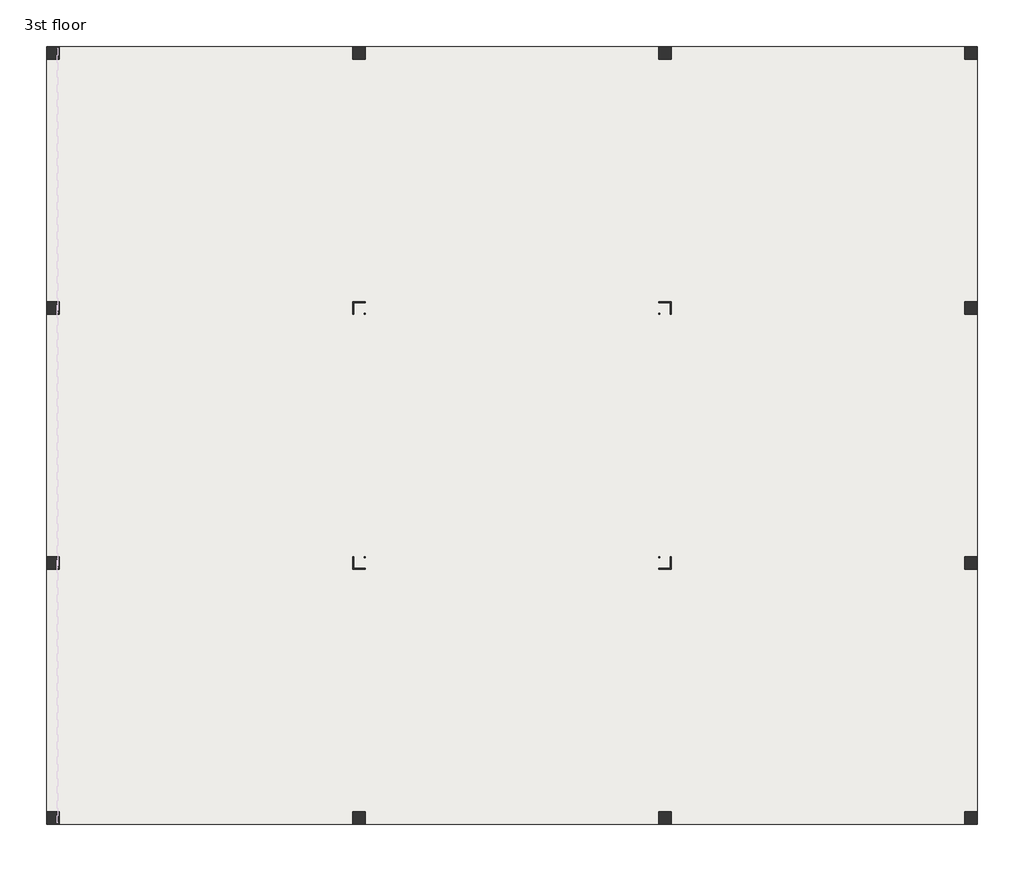
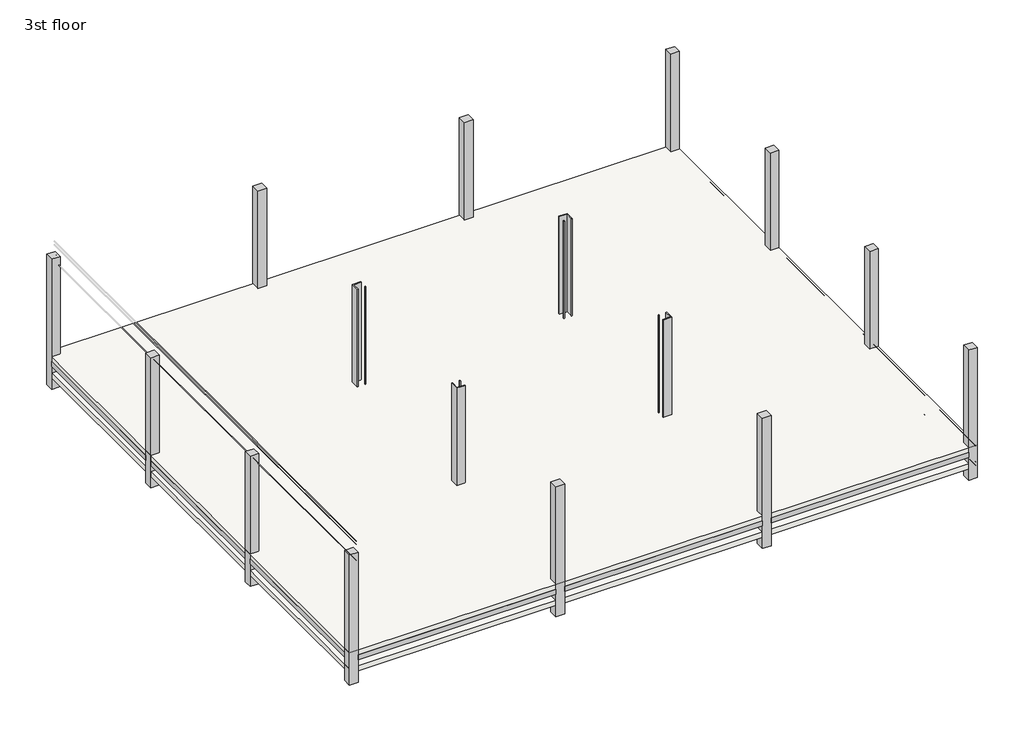
# One storey, part 1 of 2: 24 beams, 16 columns, 2 slabs.
"""IFC4 building model written with IfcOpenShell, lengths in millimetres."""

from ifc_helpers import new_model, si_unit, frame, origin, place, context, project, spatial, polyline, outline, extrude, faceted_brep, element, save

model = new_model("IFC4")

# Units and contexts
model_context = context("Model", 3, world=origin())
ifc_project = project(units=[si_unit("LENGTHUNIT", "METRE", prefix="MILLI")], contexts=[model_context])

# Site, building, storey
site = spatial("IfcSite", under=ifc_project)
building = spatial("IfcBuilding", under=site)
storey = spatial("IfcBuildingStorey", under=building, Name="3st floor", Elevation=12000.0)

# Beams
placement = place(None, origin())
element("IfcBeam", 1, ObjectType="Concrete-Rectangular Beam : 250 x 300mm", at=placement, inside=storey, context=model_context, shape_type="SweptSolid", body=[
    extrude(outline(polyline([(-8833.7181639, -5693.2383613), (-8833.7181639, -5443.2383613), (-3083.7181639, -5443.2383613), (-3083.7181639, -5693.2383613), (-8833.7181639, -5693.2383613)])), frame((0.0, 0.0, 11700.0), z_axis=(0.0, 0.0, 1.0), x_axis=(1.0, 0.0, 0.0)), (0.0, 0.0, 1.0), 150.0),
])
element("IfcBeam", 2, ObjectType="Concrete-Rectangular Beam : 250 x 300mm", at=placement, inside=storey, context=model_context, shape_type="SweptSolid", body=[
    extrude(outline(polyline([(-2833.7181639, -5693.2383613), (-2833.7181639, -5443.2383613), (2916.2818361, -5443.2383613), (2916.2818361, -5693.2383613), (-2833.7181639, -5693.2383613)])), frame((0.0, 0.0, 11700.0), z_axis=(0.0, 0.0, 1.0), x_axis=(1.0, 0.0, 0.0)), (0.0, 0.0, 1.0), 150.0),
])
element("IfcBeam", 3, ObjectType="Concrete-Rectangular Beam : 250 x 300mm", at=placement, inside=storey, context=model_context, shape_type="SweptSolid", body=[
    extrude(outline(polyline([(3166.2818361, -5693.2383613), (3166.2818361, -5443.2383613), (8916.2818361, -5443.2383613), (8916.2818361, -5693.2383613), (3166.2818361, -5693.2383613)])), frame((0.0, 0.0, 11700.0), z_axis=(0.0, 0.0, 1.0), x_axis=(1.0, 0.0, 0.0)), (0.0, 0.0, 1.0), 150.0),
])
element("IfcBeam", 4, ObjectType="Concrete-Rectangular Beam : 250 x 300mm", at=placement, inside=storey, context=model_context, shape_type="SweptSolid", body=[
    extrude(outline(polyline([(-8833.7181639, -10443.2383613), (-9083.7181639, -10443.2383613), (-9083.7181639, -5693.2383613), (-8833.7181639, -5693.2383613), (-8833.7181639, -10443.2383613)])), frame((0.0, 0.0, 11700.0), z_axis=(0.0, 0.0, 1.0), x_axis=(1.0, 0.0, 0.0)), (0.0, 0.0, 1.0), 150.0),
])
element("IfcBeam", 5, ObjectType="Concrete-Rectangular Beam : 250 x 300mm", at=placement, inside=storey, context=model_context, shape_type="SweptSolid", body=[
    extrude(outline(polyline([(-8833.7181639, -15443.2383613), (-9083.7181639, -15443.2383613), (-9083.7181639, -10693.2383613), (-8833.7181639, -10693.2383613), (-8833.7181639, -15443.2383613)])), frame((0.0, 0.0, 11700.0), z_axis=(0.0, 0.0, 1.0), x_axis=(1.0, 0.0, 0.0)), (0.0, 0.0, 1.0), 150.0),
])
element("IfcBeam", 6, ObjectType="Concrete-Rectangular Beam : 250 x 300mm", at=placement, inside=storey, context=model_context, shape_type="SweptSolid", body=[
    extrude(outline(polyline([(-8833.7181639, -20443.2383613), (-9083.7181639, -20443.2383613), (-9083.7181639, -15693.2383613), (-8833.7181639, -15693.2383613), (-8833.7181639, -20443.2383613)])), frame((0.0, 0.0, 11700.0), z_axis=(0.0, 0.0, 1.0), x_axis=(1.0, 0.0, 0.0)), (0.0, 0.0, 1.0), 150.0),
])
element("IfcBeam", 7, ObjectType="Concrete-Rectangular Beam : 250 x 300mm", at=placement, inside=storey, context=model_context, shape_type="SweptSolid", body=[
    extrude(outline(polyline([(-2833.7181639, -10443.2383613), (-3083.7181639, -10443.2383613), (-3083.7181639, -5693.2383613), (-2833.7181639, -5693.2383613), (-2833.7181639, -10443.2383613)])), frame((0.0, 0.0, 11700.0), z_axis=(0.0, 0.0, 1.0), x_axis=(1.0, 0.0, 0.0)), (0.0, 0.0, 1.0), 150.0),
])
element("IfcBeam", 8, ObjectType="Concrete-Rectangular Beam : 250 x 300mm", at=placement, inside=storey, context=model_context, shape_type="SweptSolid", body=[
    extrude(outline(polyline([(-3083.7181639, -15443.2383613), (-3083.7181639, -10693.2383613), (-3058.7181639, -10693.2383613), (-3058.7181639, -15443.2383613), (-3083.7181639, -15443.2383613)])), frame((0.0, 0.0, 11700.0), z_axis=(0.0, 0.0, 1.0), x_axis=(1.0, 0.0, 0.0)), (0.0, 0.0, 1.0), 150.0),
    extrude(outline(polyline([(-2833.7181639, -10693.2383613), (-2833.7181639, -15443.2383613), (-2858.7181639, -15443.2383613), (-2858.7181639, -10693.2383613), (-2833.7181639, -10693.2383613)])), frame((0.0, 0.0, 11700.0), z_axis=(0.0, 0.0, 1.0), x_axis=(1.0, 0.0, 0.0)), (0.0, 0.0, 1.0), 150.0),
])
element("IfcBeam", 9, ObjectType="Concrete-Rectangular Beam : 250 x 300mm", at=placement, inside=storey, context=model_context, shape_type="SweptSolid", body=[
    extrude(outline(polyline([(-2833.7181639, -20443.2383613), (-3083.7181639, -20443.2383613), (-3083.7181639, -15693.2383613), (-2833.7181639, -15693.2383613), (-2833.7181639, -20443.2383613)])), frame((0.0, 0.0, 11700.0), z_axis=(0.0, 0.0, 1.0), x_axis=(1.0, 0.0, 0.0)), (0.0, 0.0, 1.0), 150.0),
])
element("IfcBeam", 10, ObjectType="Concrete-Rectangular Beam : 250 x 300mm", at=placement, inside=storey, context=model_context, shape_type="SweptSolid", body=[
    extrude(outline(polyline([(3166.2818361, -10443.2383613), (2916.2818361, -10443.2383613), (2916.2818361, -5693.2383613), (3166.2818361, -5693.2383613), (3166.2818361, -10443.2383613)])), frame((0.0, 0.0, 11700.0), z_axis=(0.0, 0.0, 1.0), x_axis=(1.0, 0.0, 0.0)), (0.0, 0.0, 1.0), 150.0),
])
element("IfcBeam", 11, ObjectType="Concrete-Rectangular Beam : 250 x 300mm", at=placement, inside=storey, context=model_context, shape_type="SweptSolid", body=[
    extrude(outline(polyline([(2916.2818361, -15443.2383613), (2916.2818361, -10693.2383613), (2941.2818361, -10693.2383613), (2941.2818361, -15443.2383613), (2916.2818361, -15443.2383613)])), frame((0.0, 0.0, 11700.0), z_axis=(0.0, 0.0, 1.0), x_axis=(1.0, 0.0, 0.0)), (0.0, 0.0, 1.0), 150.0),
    extrude(outline(polyline([(3166.2818361, -10693.2383613), (3166.2818361, -15443.2383613), (3141.2818361, -15443.2383613), (3141.2818361, -10693.2383613), (3166.2818361, -10693.2383613)])), frame((0.0, 0.0, 11700.0), z_axis=(0.0, 0.0, 1.0), x_axis=(1.0, 0.0, 0.0)), (0.0, 0.0, 1.0), 150.0),
])
element("IfcBeam", 12, ObjectType="Concrete-Rectangular Beam : 250 x 300mm", at=placement, inside=storey, context=model_context, shape_type="SweptSolid", body=[
    extrude(outline(polyline([(3166.2818361, -20443.2383613), (2916.2818361, -20443.2383613), (2916.2818361, -15693.2383613), (3166.2818361, -15693.2383613), (3166.2818361, -20443.2383613)])), frame((0.0, 0.0, 11700.0), z_axis=(0.0, 0.0, 1.0), x_axis=(1.0, 0.0, 0.0)), (0.0, 0.0, 1.0), 150.0),
])
element("IfcBeam", 13, ObjectType="Concrete-Rectangular Beam : 250 x 300mm", at=placement, inside=storey, context=model_context, shape_type="SweptSolid", body=[
    extrude(outline(polyline([(9166.2818361, -10443.2383613), (8916.2818361, -10443.2383613), (8916.2818361, -5693.2383613), (9166.2818361, -5693.2383613), (9166.2818361, -10443.2383613)])), frame((0.0, 0.0, 11700.0), z_axis=(0.0, 0.0, 1.0), x_axis=(1.0, 0.0, 0.0)), (0.0, 0.0, 1.0), 150.0),
])
element("IfcBeam", 14, ObjectType="Concrete-Rectangular Beam : 250 x 300mm", at=placement, inside=storey, context=model_context, shape_type="SweptSolid", body=[
    extrude(outline(polyline([(9166.2818361, -15443.2383613), (8916.2818361, -15443.2383613), (8916.2818361, -10693.2383613), (9166.2818361, -10693.2383613), (9166.2818361, -15443.2383613)])), frame((0.0, 0.0, 11700.0), z_axis=(0.0, 0.0, 1.0), x_axis=(1.0, 0.0, 0.0)), (0.0, 0.0, 1.0), 150.0),
])
element("IfcBeam", 15, ObjectType="Concrete-Rectangular Beam : 250 x 300mm", at=placement, inside=storey, context=model_context, shape_type="SweptSolid", body=[
    extrude(outline(polyline([(9166.2818361, -20443.2383613), (8916.2818361, -20443.2383613), (8916.2818361, -15693.2383613), (9166.2818361, -15693.2383613), (9166.2818361, -20443.2383613)])), frame((0.0, 0.0, 11700.0), z_axis=(0.0, 0.0, 1.0), x_axis=(1.0, 0.0, 0.0)), (0.0, 0.0, 1.0), 150.0),
])
element("IfcBeam", 16, ObjectType="Concrete-Rectangular Beam : 250 x 300mm", at=placement, inside=storey, context=model_context, shape_type="SweptSolid", body=[
    extrude(outline(polyline([(-8833.7181639, -20693.2383613), (-8833.7181639, -20443.2383613), (-3083.7181639, -20443.2383613), (-3083.7181639, -20693.2383613), (-8833.7181639, -20693.2383613)])), frame((0.0, 0.0, 11700.0), z_axis=(0.0, 0.0, 1.0), x_axis=(1.0, 0.0, 0.0)), (0.0, 0.0, 1.0), 150.0),
])
element("IfcBeam", 17, ObjectType="Concrete-Rectangular Beam : 250 x 300mm", at=placement, inside=storey, context=model_context, shape_type="SweptSolid", body=[
    extrude(outline(polyline([(-2833.7181639, -20693.2383613), (-2833.7181639, -20443.2383613), (2916.2818361, -20443.2383613), (2916.2818361, -20693.2383613), (-2833.7181639, -20693.2383613)])), frame((0.0, 0.0, 11700.0), z_axis=(0.0, 0.0, 1.0), x_axis=(1.0, 0.0, 0.0)), (0.0, 0.0, 1.0), 150.0),
])
element("IfcBeam", 18, ObjectType="Concrete-Rectangular Beam : 250 x 300mm", at=placement, inside=storey, context=model_context, shape_type="SweptSolid", body=[
    extrude(outline(polyline([(3166.2818361, -20693.2383613), (3166.2818361, -20443.2383613), (8916.2818361, -20443.2383613), (8916.2818361, -20693.2383613), (3166.2818361, -20693.2383613)])), frame((0.0, 0.0, 11700.0), z_axis=(0.0, 0.0, 1.0), x_axis=(1.0, 0.0, 0.0)), (0.0, 0.0, 1.0), 150.0),
])
element("IfcBeam", 19, ObjectType="Concrete-Rectangular Beam : 250 x 300mm", at=placement, inside=storey, context=model_context, shape_type="SweptSolid", body=[
    extrude(outline(polyline([(-8833.7181639, -15693.2383613), (-8833.7181639, -15443.2383613), (-3083.7181639, -15443.2383613), (-3083.7181639, -15693.2383613), (-8833.7181639, -15693.2383613)])), frame((0.0, 0.0, 11700.0), z_axis=(0.0, 0.0, 1.0), x_axis=(1.0, 0.0, 0.0)), (0.0, 0.0, 1.0), 150.0),
])
element("IfcBeam", 20, ObjectType="Concrete-Rectangular Beam : 250 x 300mm", at=placement, inside=storey, context=model_context, shape_type="SweptSolid", body=[
    extrude(outline(polyline([(2916.2818361, -15693.2383613), (-2833.7181639, -15693.2383613), (-2833.7181639, -15668.2383613), (2916.2818361, -15668.2383613), (2916.2818361, -15693.2383613)])), frame((0.0, 0.0, 11700.0), z_axis=(0.0, 0.0, 1.0), x_axis=(1.0, 0.0, 0.0)), (0.0, 0.0, 1.0), 150.0),
    extrude(outline(polyline([(-2833.7181639, -15443.2383613), (2916.2818361, -15443.2383613), (2916.2818361, -15468.2383613), (-2833.7181639, -15468.2383613), (-2833.7181639, -15443.2383613)])), frame((0.0, 0.0, 11700.0), z_axis=(0.0, 0.0, 1.0), x_axis=(1.0, 0.0, 0.0)), (0.0, 0.0, 1.0), 150.0),
])
element("IfcBeam", 21, ObjectType="Concrete-Rectangular Beam : 250 x 300mm", at=placement, inside=storey, context=model_context, shape_type="SweptSolid", body=[
    extrude(outline(polyline([(3166.2818361, -15693.2383613), (3166.2818361, -15443.2383613), (8916.2818361, -15443.2383613), (8916.2818361, -15693.2383613), (3166.2818361, -15693.2383613)])), frame((0.0, 0.0, 11700.0), z_axis=(0.0, 0.0, 1.0), x_axis=(1.0, 0.0, 0.0)), (0.0, 0.0, 1.0), 150.0),
])
element("IfcBeam", 22, ObjectType="Concrete-Rectangular Beam : 250 x 300mm", at=placement, inside=storey, context=model_context, shape_type="SweptSolid", body=[
    extrude(outline(polyline([(-8833.7181639, -10693.2383613), (-8833.7181639, -10443.2383613), (-3083.7181639, -10443.2383613), (-3083.7181639, -10693.2383613), (-8833.7181639, -10693.2383613)])), frame((0.0, 0.0, 11700.0), z_axis=(0.0, 0.0, 1.0), x_axis=(1.0, 0.0, 0.0)), (0.0, 0.0, 1.0), 150.0),
])
element("IfcBeam", 23, ObjectType="Concrete-Rectangular Beam : 250 x 300mm", at=placement, inside=storey, context=model_context, shape_type="SweptSolid", body=[
    extrude(outline(polyline([(2916.2818361, -10693.2383613), (-2833.7181639, -10693.2383613), (-2833.7181639, -10668.2383613), (2916.2818361, -10668.2383613), (2916.2818361, -10693.2383613)])), frame((0.0, 0.0, 11700.0), z_axis=(0.0, 0.0, 1.0), x_axis=(1.0, 0.0, 0.0)), (0.0, 0.0, 1.0), 150.0),
    extrude(outline(polyline([(-2833.7181639, -10443.2383613), (2916.2818361, -10443.2383613), (2916.2818361, -10468.2383613), (-2833.7181639, -10468.2383613), (-2833.7181639, -10443.2383613)])), frame((0.0, 0.0, 11700.0), z_axis=(0.0, 0.0, 1.0), x_axis=(1.0, 0.0, 0.0)), (0.0, 0.0, 1.0), 150.0),
])
element("IfcBeam", 24, ObjectType="Concrete-Rectangular Beam : 250 x 300mm", at=placement, inside=storey, context=model_context, shape_type="SweptSolid", body=[
    extrude(outline(polyline([(3166.2818361, -10693.2383613), (3166.2818361, -10443.2383613), (8916.2818361, -10443.2383613), (8916.2818361, -10693.2383613), (3166.2818361, -10693.2383613)])), frame((0.0, 0.0, 11700.0), z_axis=(0.0, 0.0, 1.0), x_axis=(1.0, 0.0, 0.0)), (0.0, 0.0, 1.0), 150.0),
])

# Columns
element("IfcColumn", 25, ObjectType="Concrete-Rectangular-Column : 250x250 mm", at=placement, inside=storey, context=model_context, shape_type="Brep", body=[
    faceted_brep([(-8833.7181639, -20443.2383613, 15000.0), (-9083.7181639, -20443.2383613, 15000.0), (-9083.7181639, -20693.2383613, 15000.0), (-8833.7181639, -20693.2383613, 15000.0), (-8833.7181639, -20443.2383613, 11000.0), (-8833.7181639, -20693.2383613, 11000.0), (-9083.7181639, -20693.2383613, 11000.0), (-9083.7181639, -20443.2383613, 11000.0), (-8833.7181639, -20443.2383613, 11350.0), (-8833.7181639, -20443.2383613, 11200.0), (-9083.7181639, -20443.2383613, 11200.0), (-9083.7181639, -20443.2383613, 11350.0), (-8833.7181639, -20693.2383613, 11200.0), (-8833.7181639, -20693.2383613, 11350.0)], [[[0, 1, 2, 3]], [[4, 5, 6, 7]], [[1, 0, 8, 9, 4, 7, 10, 11]], [[2, 1, 11, 10, 7, 6]], [[3, 2, 6, 5, 12, 13]], [[0, 3, 13, 12, 5, 4, 9, 8]]]),
])
element("IfcColumn", 26, ObjectType="Concrete-Rectangular-Column : 250x250 mm", at=placement, inside=storey, context=model_context, shape_type="Brep", body=[
    faceted_brep([(-8833.7181639, -15443.2383613, 15000.0), (-9083.7181639, -15443.2383613, 15000.0), (-9083.7181639, -15693.2383613, 15000.0), (-8833.7181639, -15693.2383613, 15000.0), (-8833.7181639, -15443.2383613, 11000.0), (-8833.7181639, -15693.2383613, 11000.0), (-9083.7181639, -15693.2383613, 11000.0), (-9083.7181639, -15443.2383613, 11000.0), (-8833.7181639, -15443.2383613, 11350.0), (-8833.7181639, -15443.2383613, 11200.0), (-9083.7181639, -15443.2383613, 11200.0), (-9083.7181639, -15443.2383613, 11350.0), (-9083.7181639, -15693.2383613, 11200.0), (-9083.7181639, -15693.2383613, 11350.0), (-8833.7181639, -15693.2383613, 11200.0), (-8833.7181639, -15693.2383613, 11350.0)], [[[0, 1, 2, 3]], [[4, 5, 6, 7]], [[1, 0, 8, 9, 4, 7, 10, 11]], [[2, 1, 11, 10, 7, 6, 12, 13]], [[3, 2, 13, 12, 6, 5, 14, 15]], [[0, 3, 15, 14, 5, 4, 9, 8]]]),
])
element("IfcColumn", 27, ObjectType="Concrete-Rectangular-Column : 250x250 mm", at=placement, inside=storey, context=model_context, shape_type="Brep", body=[
    faceted_brep([(-8833.7181639, -10443.2383613, 15000.0), (-9083.7181639, -10443.2383613, 15000.0), (-9083.7181639, -10693.2383613, 15000.0), (-8833.7181639, -10693.2383613, 15000.0), (-8833.7181639, -10443.2383613, 11000.0), (-8833.7181639, -10693.2383613, 11000.0), (-9083.7181639, -10693.2383613, 11000.0), (-9083.7181639, -10443.2383613, 11000.0), (-8833.7181639, -10443.2383613, 11350.0), (-8833.7181639, -10443.2383613, 11200.0), (-9083.7181639, -10443.2383613, 11200.0), (-9083.7181639, -10443.2383613, 11350.0), (-9083.7181639, -10693.2383613, 11200.0), (-9083.7181639, -10693.2383613, 11350.0), (-8833.7181639, -10693.2383613, 11200.0), (-8833.7181639, -10693.2383613, 11350.0)], [[[0, 1, 2, 3]], [[4, 5, 6, 7]], [[1, 0, 8, 9, 4, 7, 10, 11]], [[2, 1, 11, 10, 7, 6, 12, 13]], [[3, 2, 13, 12, 6, 5, 14, 15]], [[0, 3, 15, 14, 5, 4, 9, 8]]]),
])
element("IfcColumn", 28, ObjectType="Concrete-Rectangular-Column : 250x250 mm", at=placement, inside=storey, context=model_context, shape_type="Brep", body=[
    faceted_brep([(-8833.7181639, -5443.2383613, 15000.0), (-9083.7181639, -5443.2383613, 15000.0), (-9083.7181639, -5693.2383613, 15000.0), (-8833.7181639, -5693.2383613, 15000.0), (-8833.7181639, -5443.2383613, 11000.0), (-8833.7181639, -5693.2383613, 11000.0), (-9083.7181639, -5693.2383613, 11000.0), (-9083.7181639, -5443.2383613, 11000.0), (-8833.7181639, -5443.2383613, 11350.0), (-8833.7181639, -5443.2383613, 11200.0), (-9083.7181639, -5693.2383613, 11200.0), (-9083.7181639, -5693.2383613, 11350.0), (-8833.7181639, -5693.2383613, 11200.0), (-8833.7181639, -5693.2383613, 11350.0)], [[[0, 1, 2, 3]], [[4, 5, 6, 7]], [[1, 0, 8, 9, 4, 7]], [[2, 1, 7, 6, 10, 11]], [[3, 2, 11, 10, 6, 5, 12, 13]], [[0, 3, 13, 12, 5, 4, 9, 8]]]),
])
element("IfcColumn", 29, ObjectType="Concrete-Rectangular-Column : 250x250 mm", at=placement, inside=storey, context=model_context, shape_type="Brep", body=[
    faceted_brep([(-2833.7181639, -20443.2383613, 15000.0), (-3083.7181639, -20443.2383613, 15000.0), (-3083.7181639, -20693.2383613, 15000.0), (-2833.7181639, -20693.2383613, 15000.0), (-2833.7181639, -20443.2383613, 11000.0), (-2833.7181639, -20693.2383613, 11000.0), (-3083.7181639, -20693.2383613, 11000.0), (-3083.7181639, -20443.2383613, 11000.0), (-2833.7181639, -20443.2383613, 11350.0), (-2833.7181639, -20443.2383613, 11200.0), (-3083.7181639, -20443.2383613, 11200.0), (-3083.7181639, -20443.2383613, 11350.0), (-3083.7181639, -20693.2383613, 11200.0), (-3083.7181639, -20693.2383613, 11350.0), (-2833.7181639, -20693.2383613, 11200.0), (-2833.7181639, -20693.2383613, 11350.0)], [[[0, 1, 2, 3]], [[4, 5, 6, 7]], [[1, 0, 8, 9, 4, 7, 10, 11]], [[2, 1, 11, 10, 7, 6, 12, 13]], [[3, 2, 13, 12, 6, 5, 14, 15]], [[0, 3, 15, 14, 5, 4, 9, 8]]]),
])
element("IfcColumn", 30, ObjectType="Concrete-Rectangular-Column : 250x250 mm", at=placement, inside=storey, context=model_context, shape_type="Brep", body=[
    faceted_brep([(-2833.7181639, -15468.2383613, 15000.0), (-2833.7181639, -15443.2383613, 15000.0), (-2858.7181639, -15443.2383613, 15000.0), (-2858.7181639, -15468.2383613, 15000.0), (-2833.7181639, -15443.2383613, 11000.0), (-2833.7181639, -15468.2383613, 11000.0), (-2858.7181639, -15468.2383613, 11000.0), (-2858.7181639, -15443.2383613, 11000.0), (-2833.7181639, -15443.2383613, 11350.0), (-2833.7181639, -15443.2383613, 11200.0), (-2858.7181639, -15443.2383613, 11200.0), (-2858.7181639, -15443.2383613, 11350.0), (-2833.7181639, -15468.2383613, 11350.0), (-2833.7181639, -15468.2383613, 11200.0)], [[[0, 1, 2, 3]], [[4, 5, 6, 7]], [[1, 8, 9, 4, 7, 10, 11, 2]], [[4, 9, 8, 1, 0, 12, 13, 5]], [[5, 13, 12, 0, 3, 6]], [[3, 2, 11, 10, 7, 6]]]),
    faceted_brep([(-3083.7181639, -15693.2383613, 15000.0), (-3083.7181639, -15443.2383613, 15000.0), (-3083.7181639, -15443.2383613, 11350.0), (-3083.7181639, -15443.2383613, 11200.0), (-3083.7181639, -15443.2383613, 11000.0), (-3083.7181639, -15693.2383613, 11000.0), (-3083.7181639, -15693.2383613, 11200.0), (-3083.7181639, -15693.2383613, 11350.0), (-2833.7181639, -15693.2383613, 15000.0), (-2833.7181639, -15693.2383613, 11000.0), (-2833.7181639, -15693.2383613, 11200.0), (-2833.7181639, -15693.2383613, 11350.0), (-3058.7181639, -15668.2383613, 11000.0), (-3058.7181639, -15668.2383613, 15000.0), (-2833.7181639, -15668.2383613, 15000.0), (-2833.7181639, -15668.2383613, 11350.0), (-2833.7181639, -15668.2383613, 11200.0), (-2833.7181639, -15668.2383613, 11000.0), (-3058.7181639, -15443.2383613, 11000.0), (-3058.7181639, -15443.2383613, 11200.0), (-3058.7181639, -15443.2383613, 11350.0), (-3058.7181639, -15443.2383613, 15000.0)], [[[0, 1, 2, 3, 4, 5, 6, 7]], [[8, 0, 7, 6, 5, 9, 10, 11]], [[12, 13, 14, 15, 16, 17]], [[13, 12, 18, 19, 20, 21]], [[8, 11, 10, 9, 17, 16, 15, 14]], [[1, 0, 8, 14, 13, 21]], [[9, 5, 4, 18, 12, 17]], [[4, 3, 2, 1, 21, 20, 19, 18]]]),
])
element("IfcColumn", 31, ObjectType="Concrete-Rectangular-Column : 250x250 mm", at=placement, inside=storey, context=model_context, shape_type="Brep", body=[
    faceted_brep([(-2833.7181639, -10443.2383613, 15000.0), (-3083.7181639, -10443.2383613, 15000.0), (-3083.7181639, -10693.2383613, 15000.0), (-3058.7181639, -10693.2383613, 15000.0), (-3058.7181639, -10468.2383613, 15000.0), (-2833.7181639, -10468.2383613, 15000.0), (-3083.7181639, -10693.2383613, 11000.0), (-3083.7181639, -10443.2383613, 11000.0), (-2833.7181639, -10443.2383613, 11000.0), (-2833.7181639, -10468.2383613, 11000.0), (-3058.7181639, -10468.2383613, 11000.0), (-3058.7181639, -10693.2383613, 11000.0), (-2833.7181639, -10443.2383613, 11350.0), (-2833.7181639, -10443.2383613, 11200.0), (-3083.7181639, -10443.2383613, 11200.0), (-3083.7181639, -10443.2383613, 11350.0), (-3083.7181639, -10693.2383613, 11200.0), (-3083.7181639, -10693.2383613, 11350.0), (-3058.7181639, -10693.2383613, 11200.0), (-3058.7181639, -10693.2383613, 11350.0), (-2833.7181639, -10468.2383613, 11350.0), (-2833.7181639, -10468.2383613, 11200.0)], [[[0, 1, 2, 3, 4, 5]], [[6, 7, 8, 9, 10, 11]], [[1, 0, 12, 13, 8, 7, 14, 15]], [[2, 1, 15, 14, 7, 6, 16, 17]], [[2, 17, 16, 6, 11, 18, 19, 3]], [[8, 13, 12, 0, 5, 20, 21, 9]], [[4, 10, 9, 21, 20, 5]], [[10, 4, 3, 19, 18, 11]]]),
    faceted_brep([(-2833.7181639, -10668.2383613, 15000.0), (-2833.7181639, -10668.2383613, 11350.0), (-2833.7181639, -10668.2383613, 11200.0), (-2833.7181639, -10668.2383613, 11000.0), (-2858.7181639, -10668.2383613, 11000.0), (-2858.7181639, -10668.2383613, 15000.0), (-2833.7181639, -10693.2383613, 15000.0), (-2833.7181639, -10693.2383613, 11350.0), (-2833.7181639, -10693.2383613, 11200.0), (-2833.7181639, -10693.2383613, 11000.0), (-2858.7181639, -10693.2383613, 15000.0), (-2858.7181639, -10693.2383613, 11000.0), (-2858.7181639, -10693.2383613, 11200.0), (-2858.7181639, -10693.2383613, 11350.0)], [[[0, 1, 2, 3, 4, 5]], [[6, 7, 8, 9, 3, 2, 1, 0]], [[10, 5, 4, 11, 12, 13]], [[6, 0, 5, 10]], [[3, 9, 11, 4]], [[9, 8, 7, 6, 10, 13, 12, 11]]]),
])
element("IfcColumn", 32, ObjectType="Concrete-Rectangular-Column : 250x250 mm", at=placement, inside=storey, context=model_context, shape_type="Brep", body=[
    faceted_brep([(-2833.7181639, -5443.2383613, 15000.0), (-3083.7181639, -5443.2383613, 15000.0), (-3083.7181639, -5693.2383613, 15000.0), (-2833.7181639, -5693.2383613, 15000.0), (-2833.7181639, -5443.2383613, 11000.0), (-2833.7181639, -5693.2383613, 11000.0), (-3083.7181639, -5693.2383613, 11000.0), (-3083.7181639, -5443.2383613, 11000.0), (-2833.7181639, -5443.2383613, 11350.0), (-2833.7181639, -5443.2383613, 11200.0), (-3083.7181639, -5443.2383613, 11200.0), (-3083.7181639, -5443.2383613, 11350.0), (-3083.7181639, -5693.2383613, 11200.0), (-3083.7181639, -5693.2383613, 11350.0), (-2833.7181639, -5693.2383613, 11200.0), (-2833.7181639, -5693.2383613, 11350.0)], [[[0, 1, 2, 3]], [[4, 5, 6, 7]], [[1, 0, 8, 9, 4, 7, 10, 11]], [[2, 1, 11, 10, 7, 6, 12, 13]], [[3, 2, 13, 12, 6, 5, 14, 15]], [[0, 3, 15, 14, 5, 4, 9, 8]]]),
])
element("IfcColumn", 33, ObjectType="Concrete-Rectangular-Column : 250x250 mm", at=placement, inside=storey, context=model_context, shape_type="Brep", body=[
    faceted_brep([(3166.2818361, -20443.2383613, 15000.0), (2916.2818361, -20443.2383613, 15000.0), (2916.2818361, -20693.2383613, 15000.0), (3166.2818361, -20693.2383613, 15000.0), (3166.2818361, -20443.2383613, 11000.0), (3166.2818361, -20693.2383613, 11000.0), (2916.2818361, -20693.2383613, 11000.0), (2916.2818361, -20443.2383613, 11000.0), (3166.2818361, -20443.2383613, 11350.0), (3166.2818361, -20443.2383613, 11200.0), (2916.2818361, -20443.2383613, 11200.0), (2916.2818361, -20443.2383613, 11350.0), (2916.2818361, -20693.2383613, 11200.0), (2916.2818361, -20693.2383613, 11350.0), (3166.2818361, -20693.2383613, 11200.0), (3166.2818361, -20693.2383613, 11350.0)], [[[0, 1, 2, 3]], [[4, 5, 6, 7]], [[1, 0, 8, 9, 4, 7, 10, 11]], [[2, 1, 11, 10, 7, 6, 12, 13]], [[3, 2, 13, 12, 6, 5, 14, 15]], [[0, 3, 15, 14, 5, 4, 9, 8]]]),
])
element("IfcColumn", 34, ObjectType="Concrete-Rectangular-Column : 250x250 mm", at=placement, inside=storey, context=model_context, shape_type="Brep", body=[
    faceted_brep([(2916.2818361, -15443.2383613, 15000.0), (2916.2818361, -15468.2383613, 15000.0), (2941.2818361, -15468.2383613, 15000.0), (2941.2818361, -15443.2383613, 15000.0), (2916.2818361, -15468.2383613, 11000.0), (2916.2818361, -15443.2383613, 11000.0), (2941.2818361, -15443.2383613, 11000.0), (2941.2818361, -15468.2383613, 11000.0), (2916.2818361, -15443.2383613, 11350.0), (2916.2818361, -15443.2383613, 11200.0), (2916.2818361, -15468.2383613, 11200.0), (2916.2818361, -15468.2383613, 11350.0), (2941.2818361, -15443.2383613, 11200.0), (2941.2818361, -15443.2383613, 11350.0)], [[[0, 1, 2, 3]], [[4, 5, 6, 7]], [[0, 8, 9, 5, 4, 10, 11, 1]], [[1, 11, 10, 4, 7, 2]], [[3, 2, 7, 6, 12, 13]], [[5, 9, 8, 0, 3, 13, 12, 6]]]),
    faceted_brep([(3166.2818361, -15443.2383613, 15000.0), (3166.2818361, -15443.2383613, 11350.0), (3166.2818361, -15443.2383613, 11200.0), (3166.2818361, -15443.2383613, 11000.0), (3141.2818361, -15443.2383613, 11000.0), (3141.2818361, -15443.2383613, 11200.0), (3141.2818361, -15443.2383613, 11350.0), (3141.2818361, -15443.2383613, 15000.0), (3166.2818361, -15693.2383613, 15000.0), (2916.2818361, -15693.2383613, 15000.0), (2916.2818361, -15693.2383613, 11350.0), (2916.2818361, -15693.2383613, 11200.0), (2916.2818361, -15693.2383613, 11000.0), (3166.2818361, -15693.2383613, 11000.0), (3166.2818361, -15693.2383613, 11200.0), (3166.2818361, -15693.2383613, 11350.0), (3141.2818361, -15668.2383613, 15000.0), (3141.2818361, -15668.2383613, 11000.0), (2916.2818361, -15668.2383613, 11000.0), (2916.2818361, -15668.2383613, 11200.0), (2916.2818361, -15668.2383613, 11350.0), (2916.2818361, -15668.2383613, 15000.0)], [[[0, 1, 2, 3, 4, 5, 6, 7]], [[8, 9, 10, 11, 12, 13, 14, 15]], [[0, 8, 15, 14, 13, 3, 2, 1]], [[16, 17, 18, 19, 20, 21]], [[17, 16, 7, 6, 5, 4]], [[12, 11, 10, 9, 21, 20, 19, 18]], [[9, 8, 0, 7, 16, 21]], [[3, 13, 12, 18, 17, 4]]]),
])
element("IfcColumn", 35, ObjectType="Concrete-Rectangular-Column : 250x250 mm", at=placement, inside=storey, context=model_context, shape_type="Brep", body=[
    faceted_brep([(3166.2818361, -10443.2383613, 15000.0), (2916.2818361, -10443.2383613, 15000.0), (2916.2818361, -10468.2383613, 15000.0), (3141.2818361, -10468.2383613, 15000.0), (3141.2818361, -10693.2383613, 15000.0), (3166.2818361, -10693.2383613, 15000.0), (3166.2818361, -10443.2383613, 11350.0), (3166.2818361, -10443.2383613, 11200.0), (3166.2818361, -10443.2383613, 11000.0), (2916.2818361, -10443.2383613, 11000.0), (2916.2818361, -10443.2383613, 11200.0), (2916.2818361, -10443.2383613, 11350.0), (2916.2818361, -10468.2383613, 11000.0), (2916.2818361, -10468.2383613, 11200.0), (2916.2818361, -10468.2383613, 11350.0), (3166.2818361, -10693.2383613, 11350.0), (3166.2818361, -10693.2383613, 11200.0), (3166.2818361, -10693.2383613, 11000.0), (3141.2818361, -10468.2383613, 11000.0), (3141.2818361, -10693.2383613, 11000.0), (3141.2818361, -10693.2383613, 11200.0), (3141.2818361, -10693.2383613, 11350.0)], [[[0, 1, 2, 3, 4, 5]], [[1, 0, 6, 7, 8, 9, 10, 11]], [[1, 11, 10, 9, 12, 13, 14, 2]], [[0, 5, 15, 16, 17, 8, 7, 6]], [[18, 3, 2, 14, 13, 12]], [[3, 18, 19, 20, 21, 4]], [[8, 17, 19, 18, 12, 9]], [[17, 16, 15, 5, 4, 21, 20, 19]]]),
    faceted_brep([(2916.2818361, -10693.2383613, 11000.0), (2916.2818361, -10668.2383613, 11000.0), (2941.2818361, -10668.2383613, 11000.0), (2941.2818361, -10693.2383613, 11000.0), (2916.2818361, -10693.2383613, 15000.0), (2916.2818361, -10693.2383613, 11350.0), (2916.2818361, -10693.2383613, 11200.0), (2941.2818361, -10693.2383613, 11200.0), (2941.2818361, -10693.2383613, 11350.0), (2941.2818361, -10693.2383613, 15000.0), (2916.2818361, -10668.2383613, 11200.0), (2916.2818361, -10668.2383613, 11350.0), (2916.2818361, -10668.2383613, 15000.0), (2941.2818361, -10668.2383613, 15000.0)], [[[0, 1, 2, 3]], [[4, 5, 6, 0, 3, 7, 8, 9]], [[1, 10, 11, 12, 13, 2]], [[0, 6, 5, 4, 12, 11, 10, 1]], [[13, 9, 8, 7, 3, 2]], [[12, 4, 9, 13]]]),
])
element("IfcColumn", 36, ObjectType="Concrete-Rectangular-Column : 250x250 mm", at=placement, inside=storey, context=model_context, shape_type="Brep", body=[
    faceted_brep([(3166.2818361, -5443.2383613, 15000.0), (2916.2818361, -5443.2383613, 15000.0), (2916.2818361, -5693.2383613, 15000.0), (3166.2818361, -5693.2383613, 15000.0), (3166.2818361, -5443.2383613, 11000.0), (3166.2818361, -5693.2383613, 11000.0), (2916.2818361, -5693.2383613, 11000.0), (2916.2818361, -5443.2383613, 11000.0), (3166.2818361, -5443.2383613, 11350.0), (3166.2818361, -5443.2383613, 11200.0), (2916.2818361, -5443.2383613, 11200.0), (2916.2818361, -5443.2383613, 11350.0), (2916.2818361, -5693.2383613, 11200.0), (2916.2818361, -5693.2383613, 11350.0), (3166.2818361, -5693.2383613, 11200.0), (3166.2818361, -5693.2383613, 11350.0)], [[[0, 1, 2, 3]], [[4, 5, 6, 7]], [[1, 0, 8, 9, 4, 7, 10, 11]], [[2, 1, 11, 10, 7, 6, 12, 13]], [[3, 2, 13, 12, 6, 5, 14, 15]], [[0, 3, 15, 14, 5, 4, 9, 8]]]),
])
element("IfcColumn", 37, ObjectType="Concrete-Rectangular-Column : 250x250 mm", at=placement, inside=storey, context=model_context, shape_type="Brep", body=[
    faceted_brep([(9166.2818361, -20443.2383613, 15000.0), (8916.2818361, -20443.2383613, 15000.0), (8916.2818361, -20693.2383613, 15000.0), (9166.2818361, -20693.2383613, 15000.0), (9166.2818361, -20443.2383613, 11000.0), (9166.2818361, -20693.2383613, 11000.0), (8916.2818361, -20693.2383613, 11000.0), (8916.2818361, -20443.2383613, 11000.0), (9166.2818361, -20443.2383613, 11350.0), (9166.2818361, -20443.2383613, 11200.0), (8916.2818361, -20443.2383613, 11200.0), (8916.2818361, -20443.2383613, 11350.0), (8916.2818361, -20693.2383613, 11200.0), (8916.2818361, -20693.2383613, 11350.0)], [[[0, 1, 2, 3]], [[4, 5, 6, 7]], [[1, 0, 8, 9, 4, 7, 10, 11]], [[2, 1, 11, 10, 7, 6, 12, 13]], [[3, 2, 13, 12, 6, 5]], [[0, 3, 5, 4, 9, 8]]]),
])
element("IfcColumn", 38, ObjectType="Concrete-Rectangular-Column : 250x250 mm", at=placement, inside=storey, context=model_context, shape_type="Brep", body=[
    faceted_brep([(9166.2818361, -15443.2383613, 15000.0), (8916.2818361, -15443.2383613, 15000.0), (8916.2818361, -15693.2383613, 15000.0), (9166.2818361, -15693.2383613, 15000.0), (9166.2818361, -15443.2383613, 11000.0), (9166.2818361, -15693.2383613, 11000.0), (8916.2818361, -15693.2383613, 11000.0), (8916.2818361, -15443.2383613, 11000.0), (9166.2818361, -15443.2383613, 11350.0), (9166.2818361, -15443.2383613, 11200.0), (8916.2818361, -15443.2383613, 11200.0), (8916.2818361, -15443.2383613, 11350.0), (8916.2818361, -15693.2383613, 11200.0), (8916.2818361, -15693.2383613, 11350.0), (9166.2818361, -15693.2383613, 11200.0), (9166.2818361, -15693.2383613, 11350.0)], [[[0, 1, 2, 3]], [[4, 5, 6, 7]], [[1, 0, 8, 9, 4, 7, 10, 11]], [[2, 1, 11, 10, 7, 6, 12, 13]], [[3, 2, 13, 12, 6, 5, 14, 15]], [[0, 3, 15, 14, 5, 4, 9, 8]]]),
])
element("IfcColumn", 39, ObjectType="Concrete-Rectangular-Column : 250x250 mm", at=placement, inside=storey, context=model_context, shape_type="Brep", body=[
    faceted_brep([(9166.2818361, -10443.2383613, 15000.0), (8916.2818361, -10443.2383613, 15000.0), (8916.2818361, -10693.2383613, 15000.0), (9166.2818361, -10693.2383613, 15000.0), (9166.2818361, -10443.2383613, 11000.0), (9166.2818361, -10693.2383613, 11000.0), (8916.2818361, -10693.2383613, 11000.0), (8916.2818361, -10443.2383613, 11000.0), (9166.2818361, -10443.2383613, 11350.0), (9166.2818361, -10443.2383613, 11200.0), (8916.2818361, -10443.2383613, 11200.0), (8916.2818361, -10443.2383613, 11350.0), (8916.2818361, -10693.2383613, 11200.0), (8916.2818361, -10693.2383613, 11350.0), (9166.2818361, -10693.2383613, 11200.0), (9166.2818361, -10693.2383613, 11350.0)], [[[0, 1, 2, 3]], [[4, 5, 6, 7]], [[1, 0, 8, 9, 4, 7, 10, 11]], [[2, 1, 11, 10, 7, 6, 12, 13]], [[3, 2, 13, 12, 6, 5, 14, 15]], [[0, 3, 15, 14, 5, 4, 9, 8]]]),
])
element("IfcColumn", 40, ObjectType="Concrete-Rectangular-Column : 250x250 mm", at=placement, inside=storey, context=model_context, shape_type="Brep", body=[
    faceted_brep([(9166.2818361, -5443.2383613, 15000.0), (8916.2818361, -5443.2383613, 15000.0), (8916.2818361, -5693.2383613, 15000.0), (9166.2818361, -5693.2383613, 15000.0), (9166.2818361, -5443.2383613, 11000.0), (9166.2818361, -5693.2383613, 11000.0), (8916.2818361, -5693.2383613, 11000.0), (8916.2818361, -5443.2383613, 11000.0), (8916.2818361, -5443.2383613, 11200.0), (8916.2818361, -5443.2383613, 11350.0), (8916.2818361, -5693.2383613, 11200.0), (8916.2818361, -5693.2383613, 11350.0), (9166.2818361, -5693.2383613, 11200.0), (9166.2818361, -5693.2383613, 11350.0)], [[[0, 1, 2, 3]], [[4, 5, 6, 7]], [[1, 0, 4, 7, 8, 9]], [[2, 1, 9, 8, 7, 6, 10, 11]], [[3, 2, 11, 10, 6, 5, 12, 13]], [[0, 3, 13, 12, 5, 4]]]),
])

# Slabs
element("IfcSlab", 41, ObjectType="150mm Foundation Slab", at=placement, inside=storey, context=model_context, shape_type="Brep", body=[
    faceted_brep([(-9083.7181639, -5443.2383613, 11350.0), (-8833.7181639, -5443.2383613, 11350.0), (-3083.7181639, -5443.2383613, 11350.0), (-2833.7181639, -5443.2383613, 11350.0), (2916.2818361, -5443.2383613, 11350.0), (3166.2818361, -5443.2383613, 11350.0), (8916.2818361, -5443.2383613, 11350.0), (9166.2818361, -5443.2383613, 11350.0), (9166.2818361, -5693.2383613, 11350.0), (9166.2818361, -10443.2383613, 11350.0), (9166.2818361, -10693.2383613, 11350.0), (9166.2818361, -15443.2383613, 11350.0), (9166.2818361, -15693.2383613, 11350.0), (9166.2818361, -20443.2383613, 11350.0), (9166.2818361, -20693.2383613, 11350.0), (8916.2818361, -20693.2383613, 11350.0), (3166.2818361, -20693.2383613, 11350.0), (2916.2818361, -20693.2383613, 11350.0), (-2833.7181639, -20693.2383613, 11350.0), (-3083.7181639, -20693.2383613, 11350.0), (-8833.7181639, -20693.2383613, 11350.0), (-9083.7181639, -20693.2383613, 11350.0), (-9083.7181639, -20443.2383613, 11350.0), (-9083.7181639, -15693.2383613, 11350.0), (-9083.7181639, -15443.2383613, 11350.0), (-9083.7181639, -10693.2383613, 11350.0), (-9083.7181639, -10443.2383613, 11350.0), (-9083.7181639, -5693.2383613, 11350.0), (-9083.7181639, -5443.2383613, 11500.0), (-9083.7181639, -20693.2383613, 11500.0), (9166.2818361, -20693.2383613, 11500.0), (9166.2818361, -5443.2383613, 11500.0)], [[[0, 1, 2, 3, 4, 5, 6, 7, 8, 9, 10, 11, 12, 13, 14, 15, 16, 17, 18, 19, 20, 21, 22, 23, 24, 25, 26, 27]], [[28, 29, 30, 31]], [[7, 6, 5, 4, 3, 2, 1, 0, 28, 31]], [[14, 13, 12, 11, 10, 9, 8, 7, 31, 30]], [[21, 20, 19, 18, 17, 16, 15, 14, 30, 29]], [[0, 27, 26, 25, 24, 23, 22, 21, 29, 28]]]),
])
element("IfcSlab", 42, ObjectType="150mm Foundation Slab", at=placement, inside=storey, context=model_context, shape_type="Brep", body=[
    faceted_brep([(-9083.7181639, -5443.2383613, 11850.0), (-8833.7181639, -5443.2383613, 11850.0), (-3083.7181639, -5443.2383613, 11850.0), (-2833.7181639, -5443.2383613, 11850.0), (2916.2818361, -5443.2383613, 11850.0), (3166.2818361, -5443.2383613, 11850.0), (8916.2818361, -5443.2383613, 11850.0), (9166.2818361, -5443.2383613, 11850.0), (9166.2818361, -5693.2383613, 11850.0), (9166.2818361, -10443.2383613, 11850.0), (9166.2818361, -10693.2383613, 11850.0), (9166.2818361, -15443.2383613, 11850.0), (9166.2818361, -15693.2383613, 11850.0), (9166.2818361, -20443.2383613, 11850.0), (9166.2818361, -20693.2383613, 11850.0), (8916.2818361, -20693.2383613, 11850.0), (3166.2818361, -20693.2383613, 11850.0), (2916.2818361, -20693.2383613, 11850.0), (-2833.7181639, -20693.2383613, 11850.0), (-3083.7181639, -20693.2383613, 11850.0), (-8833.7181639, -20693.2383613, 11850.0), (-9083.7181639, -20693.2383613, 11850.0), (-9083.7181639, -20443.2383613, 11850.0), (-9083.7181639, -15693.2383613, 11850.0), (-9083.7181639, -15443.2383613, 11850.0), (-9083.7181639, -10693.2383613, 11850.0), (-9083.7181639, -10443.2383613, 11850.0), (-9083.7181639, -5693.2383613, 11850.0), (-9083.7181639, -5443.2383613, 12000.0), (-9083.7181639, -20693.2383613, 12000.0), (9166.2818361, -20693.2383613, 12000.0), (9166.2818361, -5443.2383613, 12000.0)], [[[0, 1, 2, 3, 4, 5, 6, 7, 8, 9, 10, 11, 12, 13, 14, 15, 16, 17, 18, 19, 20, 21, 22, 23, 24, 25, 26, 27]], [[28, 29, 30, 31]], [[7, 6, 5, 4, 3, 2, 1, 0, 28, 31]], [[14, 13, 12, 11, 10, 9, 8, 7, 31, 30]], [[21, 20, 19, 18, 17, 16, 15, 14, 30, 29]], [[0, 27, 26, 25, 24, 23, 22, 21, 29, 28]]]),
])

save(model, "model.ifc")

# Revit data of these elements
# Type "Concrete-Rectangular Beam : 250 x 300mm"
#   Length [instance default] = 1524 mm
#   b = 250 mm
#   h = 300 mm
#   Structural Material [instance default] = Concrete, Cast-in-Place gray
#   Assembly Code = ""
# Type "Concrete-Rectangular-Column : 250x250 mm"
#   b = 250 mm
#   h = 250 mm
#   Structural Material [instance default] = Concrete, Cast-in-Place gray
# Type "150mm Foundation Slab"
#   Layers, outside or top first: 150 mm "Concrete, Cast-in-Place gray" (function 1)
# Elements 1, 2, 3, 4, 5, 6, 7, 8, 9, 10, 11, 12, 13, 14, 15, 16, 17, 18, 19, 20, 21, 22, 23, 24 (IfcBeam, "Concrete-Rectangular Beam : 250 x 300mm")
#   Structural Material = Concrete, Cast-in-Place gray
#   Phase Created = New Construction
#   Materials on its faces: "Concrete, Cast-in-Place gray"
# Elements 25, 26, 27, 28, 29, 30, 31, 32, 33, 34, 35, 36, 37, 38, 39, 40 (IfcColumn, "Concrete-Rectangular-Column : 250x250 mm")
#   Structural Material = Concrete, Cast-in-Place gray
#   Phase Created = New Construction
#   Materials on its faces: "Concrete, Cast-in-Place gray"
# Element 41 (IfcSlab, "150mm Foundation Slab")
#   built-in parameter 1001955 = 3.14159 (stored number, unit not read)
#   Height Offset From Level = -500 mm
#   built-in parameter 1001954 = 1
#   Phase Created = New Construction
#   Materials on its faces: "Concrete, Cast-in-Place gray"
# Element 42 (IfcSlab, "150mm Foundation Slab")
#   built-in parameter 1001955 = 3.14159 (stored number, unit not read)
#   Height Offset From Level = 0 mm
#   built-in parameter 1001954 = 1
#   Phase Created = New Construction
#   Materials on its faces: "Concrete, Cast-in-Place gray"
# Materials
#   "Concrete, Cast-in-Place gray": class "Concrete", colour RGB 192 192 192, transparency 0, Description = "Cast-in-place concrete", Cost = 0
